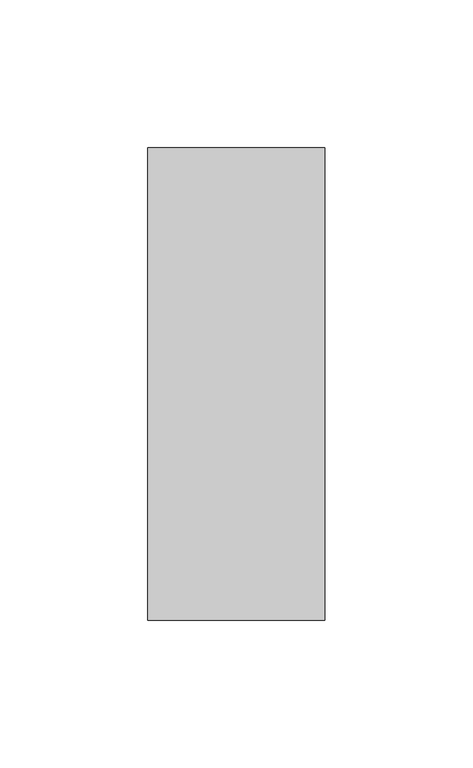
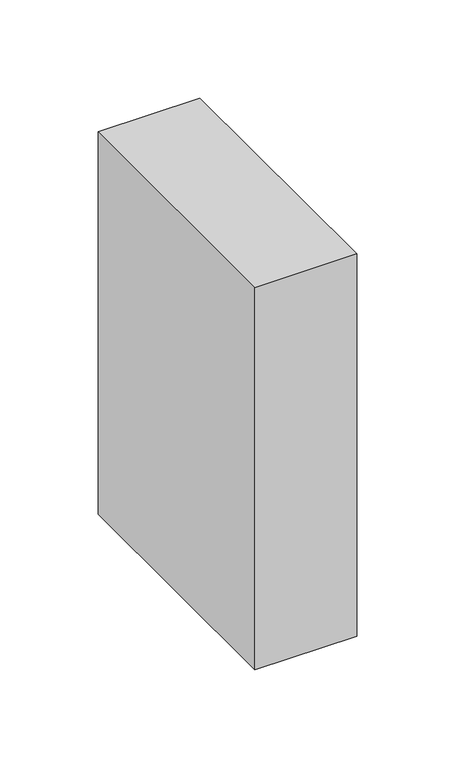
"""IFC4 building model written with IfcOpenShell, lengths in millimetres: column geometry, Madeira de lei-Coluna : Pontalete 6X16cm."""

import ifcopenshell
import ifcopenshell.guid

model = None  # the IFC model being written
_history = None  # IfcOwnerHistory: only IFC2X3 demands one
_inside = {}  # id of a spatial element -> (the spatial element, [elements in it])
_under = {}  # id of a project, library or spatial element -> (it, [spatial elements below it])
_declared = {}  # id of a project -> (the project, [libraries it declares])
_typed = {}  # id of a type object -> (the type object, [elements of that type])
_made_of = {}  # id of a material, layer set ... -> (it, [elements and type objects made of it])


def new_model(schema):
    """Start an empty IFC model of exactly this schema.

    Asked for "IFC4X3", IfcOpenShell would pick the latest addendum, in which some entities
    have other attributes; the version numbers below select the first issue.
    IFC2X3 requires an IfcOwnerHistory on every rooted entity: one is made here for all.
    """
    global model, _history
    if schema == "IFC4X3":
        model = ifcopenshell.file(schema_version=(4, 3, 0, 0))
    else:
        model = ifcopenshell.file(schema=schema)
    _inside.clear()
    _under.clear()
    _declared.clear()
    _typed.clear()
    _made_of.clear()
    _history = None
    if model.schema == "IFC2X3":
        org = make("IfcOrganization", Name="unknown")
        user = make(
            "IfcPersonAndOrganization",
            ThePerson=make("IfcPerson", FamilyName="unknown"),
            TheOrganization=org,
        )
        app = make(
            "IfcApplication",
            ApplicationDeveloper=org,
            Version="unknown",
            ApplicationFullName="unknown",
            ApplicationIdentifier="unknown",
        )
        _history = make(
            "IfcOwnerHistory",
            OwningUser=user,
            OwningApplication=app,
            ChangeAction="ADDED",
            CreationDate=0,
        )
    return model


def make(cls, **values):
    """One entity of the class cls with the attributes given. An attribute that is None is left unset."""
    return model.create_entity(
        cls, **{name: value for name, value in values.items() if value is not None}
    )


def rooted(cls, **values):
    """An entity with a GlobalId (a new one), such as an element, a storey or a relation."""
    return make(cls, GlobalId=ifcopenshell.guid.new(), OwnerHistory=_history, **values)


def si_unit(unit_type, name, prefix=None):
    """IfcSIUnit, for example si_unit("LENGTHUNIT", "METRE", prefix="MILLI")."""
    return make("IfcSIUnit", UnitType=unit_type, Prefix=prefix, Name=name)


def assignment(units):
    """IfcUnitAssignment: the units of a project."""
    return None if units is None else make("IfcUnitAssignment", Units=units)


def point(xyz):
    """IfcCartesianPoint."""
    return None if xyz is None else make("IfcCartesianPoint", Coordinates=xyz)


def direction(xyz):
    """IfcDirection."""
    return None if xyz is None else make("IfcDirection", DirectionRatios=xyz)


def frame(location, z_axis=None, x_axis=None):
    """IfcAxis2Placement3D, a coordinate frame: its origin and axes. An axis left out is left unset."""
    return make(
        "IfcAxis2Placement3D",
        Location=point(location),
        Axis=direction(z_axis),
        RefDirection=direction(x_axis),
    )


def origin():
    """The frame at (0, 0, 0) with its axes left unset."""
    return frame((0.0, 0.0, 0.0))


def place(relative_to, where):
    """IfcLocalPlacement: puts the frame where relative to a parent placement (None: the world)."""
    return make(
        "IfcLocalPlacement", PlacementRelTo=relative_to, RelativePlacement=where
    )


def context(
    kind, dimensions, precision=None, world=None, true_north=None, identifier=None
):
    """IfcGeometricRepresentationContext, for example the 3D "Model" context."""
    return make(
        "IfcGeometricRepresentationContext",
        ContextIdentifier=identifier,
        ContextType=kind,
        CoordinateSpaceDimension=dimensions,
        Precision=precision,
        WorldCoordinateSystem=world,
        TrueNorth=true_north,
    )


def project(units=None, contexts=None):
    """IfcProject with its units and contexts."""
    return rooted(
        "IfcProject",
        Name="project",
        RepresentationContexts=contexts,
        UnitsInContext=assignment(units),
    )


def spatial(cls, under=None, at=None, **own):
    """A site, building, storey or space (cls), placed at a placement, below another one or the project."""
    s = rooted(cls, ObjectPlacement=at, **own)
    if under is not None:
        _under.setdefault(under.id(), (under, []))[1].append(s)
    return s


def polyline(points):
    """IfcPolyline through the points."""
    return make("IfcPolyline", Points=[point(p) for p in points])


def outline(outer, holes=None, kind="AREA"):
    """IfcArbitraryClosedProfileDef: a profile drawn as a closed curve; with holes, ...WithVoids."""
    if holes is None:
        return make("IfcArbitraryClosedProfileDef", ProfileType=kind, OuterCurve=outer)
    return make(
        "IfcArbitraryProfileDefWithVoids",
        ProfileType=kind,
        OuterCurve=outer,
        InnerCurves=holes,
    )


def extrude(swept, where, along, depth):
    """IfcExtrudedAreaSolid: the profile swept, set in the frame where, extruded along a direction by depth."""
    return make(
        "IfcExtrudedAreaSolid",
        SweptArea=swept,
        Position=where,
        ExtrudedDirection=direction(along),
        Depth=depth,
    )


def shape(context_of_items, identifier, shape_type, items):
    """IfcShapeRepresentation: the items that make up one representation, for example the "Body"."""
    return make(
        "IfcShapeRepresentation",
        ContextOfItems=context_of_items,
        RepresentationIdentifier=identifier,
        RepresentationType=shape_type,
        Items=items,
    )


def source(mapping_origin, context_of_items, identifier, shape_type, items):
    """IfcRepresentationMap: a shape defined once, which mapped items show again and again."""
    return make(
        "IfcRepresentationMap",
        MappingOrigin=mapping_origin,
        MappedRepresentation=shape(context_of_items, identifier, shape_type, items),
    )


def transform(
    local_origin,
    x_axis=None,
    y_axis=None,
    z_axis=None,
    scale=None,
    scale2=None,
    scale3=None,
    uniform=True,
):
    """IfcCartesianTransformationOperator3D, or its non-uniform kind. x_axis, y_axis, z_axis: its Axis1, 2, 3."""
    if uniform:
        return make(
            "IfcCartesianTransformationOperator3D",
            Axis1=direction(x_axis),
            Axis2=direction(y_axis),
            LocalOrigin=point(local_origin),
            Scale=scale,
            Axis3=direction(z_axis),
        )
    return make(
        "IfcCartesianTransformationOperator3DnonUniform",
        Axis1=direction(x_axis),
        Axis2=direction(y_axis),
        LocalOrigin=point(local_origin),
        Scale=scale,
        Axis3=direction(z_axis),
        Scale2=scale2,
        Scale3=scale3,
    )


def mapped(mapping_source, mapping_target):
    """IfcMappedItem: shows the shape of a source again, moved by a transform."""
    return make(
        "IfcMappedItem", MappingSource=mapping_source, MappingTarget=mapping_target
    )


def made_of(thing, what):
    """Note that an element or type object is made of a material, layer set ...; save() writes the relation."""
    if what is not None:
        _made_of.setdefault(what.id(), (what, []))[1].append(thing)
    return thing


def element(
    cls,
    number,
    at=None,
    inside=None,
    cuts=None,
    type_object=None,
    material=None,
    context=None,
    identifier="Body",
    shape_type=None,
    held_by="IfcProductDefinitionShape",
    body=None,
    shapes=None,
    **own,
):
    """One element of the class cls, such as IfcWall. Its Tag is "e" and its number.

    at: its placement. inside: the storey or other place that contains it. cuts: it is an
    opening in that element (IfcRelVoidsElement). A single representation is given by context,
    identifier, shape_type and body (its items); several are given by shapes. held_by: the class
    of the entity that holds the representations. save() writes the other relations.
    """
    e = rooted(cls, Tag="e%d" % number, ObjectPlacement=at, **own)
    if body is not None:
        shapes = [shape(context, identifier, shape_type, body)]
    if shapes is not None:
        e.Representation = make(held_by, Representations=shapes)
    if inside is not None:
        _inside.setdefault(inside.id(), (inside, []))[1].append(e)
    if cuts is not None:
        rooted(
            "IfcRelVoidsElement", RelatingBuildingElement=cuts, RelatedOpeningElement=e
        )
    if type_object is not None:
        _typed.setdefault(type_object.id(), (type_object, []))[1].append(e)
    return made_of(e, material)


def aggregate(whole, parts):
    """IfcRelAggregates: a whole, such as a stair, and the parts it consists of."""
    return rooted("IfcRelAggregates", RelatingObject=whole, RelatedObjects=parts)


def save(model, path):
    """Write the relations noted so far, then the file.

    IfcRelAggregates (storeys below a building ...), IfcRelContainedInSpatialStructure (elements
    in a storey), IfcRelDefinesByType, IfcRelAssociatesMaterial and IfcRelDeclares: one each for
    every whole, place, type object, material and project.
    """
    for whole, parts in _under.values():
        aggregate(whole, parts)
    for where, things in _inside.values():
        rooted(
            "IfcRelContainedInSpatialStructure",
            RelatedElements=things,
            RelatingStructure=where,
        )
    for kind, things in _typed.values():
        rooted("IfcRelDefinesByType", RelatedObjects=things, RelatingType=kind)
    for what, things in _made_of.values():
        rooted("IfcRelAssociatesMaterial", RelatedObjects=things, RelatingMaterial=what)
    for by, libraries in _declared.values():
        rooted("IfcRelDeclares", RelatingContext=by, RelatedDefinitions=libraries)
    model.write(path)


def column_1cffec27(model_context):
    return source(origin(), model_context, "Body", "SweptSolid", [
        extrude(outline(polyline([(30.0, 80.0), (30.0, -80.0), (-30.0, -80.0), (-30.0, 80.0), (30.0, 80.0)])), frame((0.0, 0.0, 3110.0), z_axis=(0.0, 0.0, 1.0), x_axis=(1.0, 0.0, 0.0)), (0.0, 0.0, 1.0), 238.0),
    ])


if __name__ == "__main__":
    model = new_model("IFC4")
    model_context = context("Model", 3, world=origin())
    ifc_project = project(units=[si_unit("LENGTHUNIT", "METRE", prefix="MILLI")], contexts=[model_context])
    site = spatial("IfcSite", under=ifc_project)
    building = spatial("IfcBuilding", under=site)
    placement = place(None, origin())
    column_shape = column_1cffec27(model_context)
    element("IfcColumn", 1, ObjectType="Madeira de lei-Coluna : Pontalete 6X16cm", at=placement, inside=building, context=model_context, shape_type="MappedRepresentation", body=[
        mapped(column_shape, transform((0.0, 0.0, 0.0), x_axis=(1.0, 0.0, 0.0), y_axis=(0.0, 1.0, 0.0), z_axis=(0.0, 0.0, 1.0))),
    ])
    save(model, "model.ifc")

# Revit data of these elements
# Project information
#   Design Option = "Main Model"
#   Project Status = "Status do projeto"
#   Project Address = "RUA SÉRGIO DIAS, LOTE 30, QUADRA G, MONTE MINEIRO/MG"
#   Project Name = "RESIDÊNCIA - ROBERTA VENDRAMINI"
#   Project Number = "034/2017"
#   Zona = "ZER - 01"
#   CA Mín = "0.2"
#   CA Básico = "1"
#   CA Máx = "2"
#   TO Máx = "50"
#   Gabarito Máx = "10"
#   TP Mín = "15"
#   Área Total do Terreno = "620.00 m²"
#   Multifamiliar - Vagas Veículos/Pavto = "0"
#   Multifamiliar - Vagas Bicicletas/Pavto = "0"
#   Multifamiliar - % Vagas PNMR = "0"
#   Multifamiliar - % Vagas Motos = "0"
#   Outros - Área p/ 1 Veículo = "0.00 m²"
#   Outros - Área p/ 1 Bicicleta = "0.00 m²"
#   Outros - Área p/ 1 Utilitário = "0.00 m²"
#   Outros - % Vagas PNMR = "0"
#   Outros - % Vagas Motos = "0"
# Type "Madeira de lei-Coluna : Pontalete 6X16cm"
#   A = 0.01952 m²
#   b = 0.06 m
#   d = 0.16 m
#   Structural Material [instance default] = none
#   Assembly Code = ""
# Element 1 (IfcColumn, "Madeira de lei-Coluna : Pontalete 6X16cm")
#   Structural Material = .MADEIRAMENTO
#   Materials on its faces: ".MADEIRAMENTO"
# Materials
#   ".MADEIRAMENTO": class ".CC_MADEIRAS", colour RGB 212 179 113, transparency 0, Cost = 0
